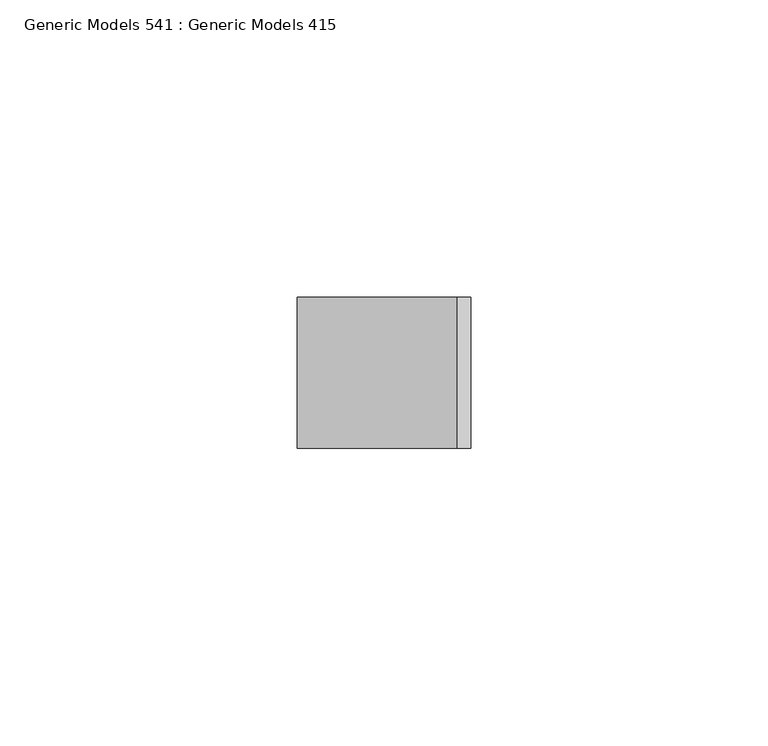
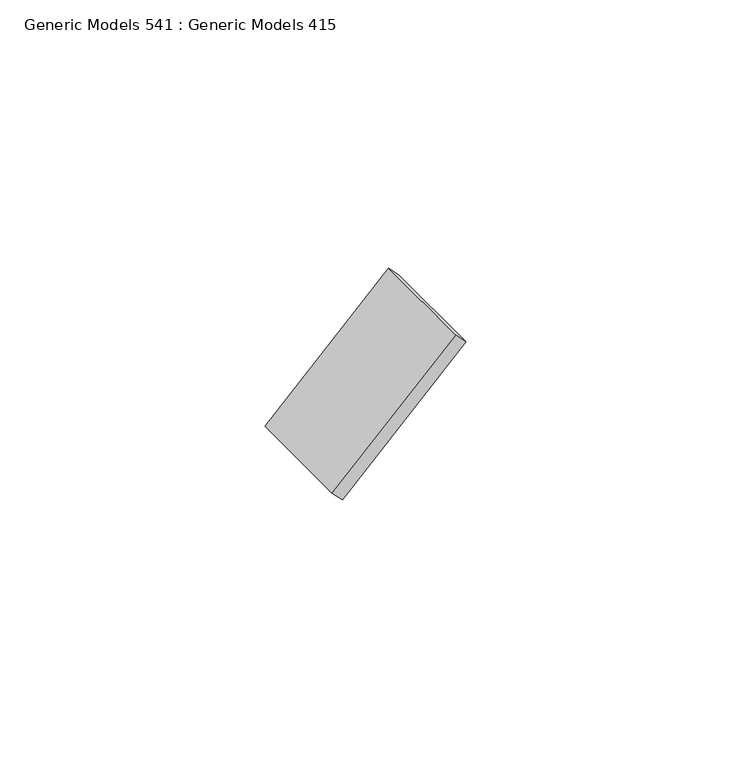
"""IFC4 building model written with IfcOpenShell, lengths in millimetres: proxy geometry, Generic Models 541 : Generic Models 415."""

from ifc_helpers import new_model, si_unit, frame, origin, place, context, project, spatial, polyline, outline, extrude, source, transform, mapped, element, save


def generic_models_541_generic_models_415_c24f0881(model_context):
    return source(origin(), model_context, "Body", "SweptSolid", [
        extrude(outline(polyline([(0.0, -3.175), (0.0, 0.0), (25.4, 0.0), (25.4, -3.175), (0.0, -3.175)])), frame((7848.0411784, 4501.3863946, 125003.8849742), z_axis=(0.7071067811867181, 0.0, 0.707106781186377), x_axis=(0.0, -1.0, 0.0)), (0.0, 0.0, 1.0), 38.1),
    ])


if __name__ == "__main__":
    model = new_model("IFC4")
    model_context = context("Model", 3, world=origin())
    ifc_project = project(units=[si_unit("LENGTHUNIT", "METRE", prefix="MILLI")], contexts=[model_context])
    site = spatial("IfcSite", under=ifc_project)
    building = spatial("IfcBuilding", under=site)
    placement = place(None, origin())
    generic_models_541_generic_models_415_shape = generic_models_541_generic_models_415_c24f0881(model_context)
    element("IfcBuildingElementProxy", 1, Name="Generic Models 541 : Generic Models 415", ObjectType="Generic Models 541 : Generic Models 415", at=placement, inside=building, context=model_context, shape_type="MappedRepresentation", body=[
        mapped(generic_models_541_generic_models_415_shape, transform((0.0, 0.0, 0.0), x_axis=(1.0, 0.0, 0.0), y_axis=(0.0, 1.0, 0.0), z_axis=(0.0, 0.0, 1.0))),
    ])
    save(model, "model.ifc")

# Revit data of these elements
# Element 1 (IfcBuildingElementProxy, "Generic Models 541 : Generic Models 415")
#   Materials on its faces: "_WELDED STEEL TABS FOR LOUVER ATTACHMENT"
# Materials
#   "_WELDED STEEL TABS FOR LOUVER ATTACHMENT": class "Metal", colour RGB 199 199 199, transparency 0, Description = "Structural steel 50ksi", Cost = 0
